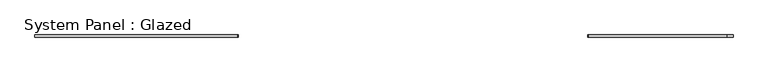
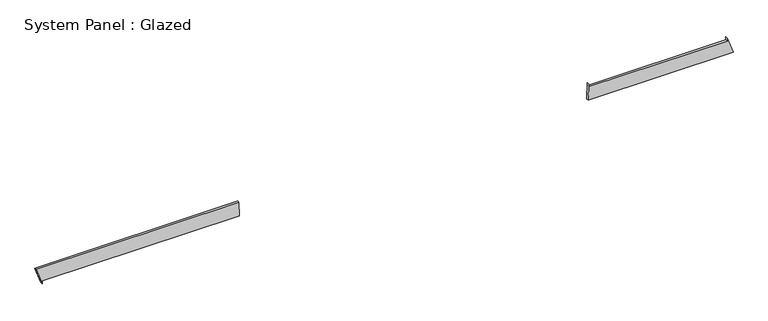
"""IFC4 building model written with IfcOpenShell, lengths in millimetres: plate geometry, System Panel : Glazed."""

import ifcopenshell
import ifcopenshell.guid

model = None  # the IFC model being written
_history = None  # IfcOwnerHistory: only IFC2X3 demands one
_inside = {}  # id of a spatial element -> (the spatial element, [elements in it])
_under = {}  # id of a project, library or spatial element -> (it, [spatial elements below it])
_declared = {}  # id of a project -> (the project, [libraries it declares])
_typed = {}  # id of a type object -> (the type object, [elements of that type])
_made_of = {}  # id of a material, layer set ... -> (it, [elements and type objects made of it])


def new_model(schema):
    """Start an empty IFC model of exactly this schema.

    Asked for "IFC4X3", IfcOpenShell would pick the latest addendum, in which some entities
    have other attributes; the version numbers below select the first issue.
    IFC2X3 requires an IfcOwnerHistory on every rooted entity: one is made here for all.
    """
    global model, _history
    if schema == "IFC4X3":
        model = ifcopenshell.file(schema_version=(4, 3, 0, 0))
    else:
        model = ifcopenshell.file(schema=schema)
    _inside.clear()
    _under.clear()
    _declared.clear()
    _typed.clear()
    _made_of.clear()
    _history = None
    if model.schema == "IFC2X3":
        org = make("IfcOrganization", Name="unknown")
        user = make(
            "IfcPersonAndOrganization",
            ThePerson=make("IfcPerson", FamilyName="unknown"),
            TheOrganization=org,
        )
        app = make(
            "IfcApplication",
            ApplicationDeveloper=org,
            Version="unknown",
            ApplicationFullName="unknown",
            ApplicationIdentifier="unknown",
        )
        _history = make(
            "IfcOwnerHistory",
            OwningUser=user,
            OwningApplication=app,
            ChangeAction="ADDED",
            CreationDate=0,
        )
    return model


def make(cls, **values):
    """One entity of the class cls with the attributes given. An attribute that is None is left unset."""
    return model.create_entity(
        cls, **{name: value for name, value in values.items() if value is not None}
    )


def rooted(cls, **values):
    """An entity with a GlobalId (a new one), such as an element, a storey or a relation."""
    return make(cls, GlobalId=ifcopenshell.guid.new(), OwnerHistory=_history, **values)


def si_unit(unit_type, name, prefix=None):
    """IfcSIUnit, for example si_unit("LENGTHUNIT", "METRE", prefix="MILLI")."""
    return make("IfcSIUnit", UnitType=unit_type, Prefix=prefix, Name=name)


def assignment(units):
    """IfcUnitAssignment: the units of a project."""
    return None if units is None else make("IfcUnitAssignment", Units=units)


def point(xyz):
    """IfcCartesianPoint."""
    return None if xyz is None else make("IfcCartesianPoint", Coordinates=xyz)


def direction(xyz):
    """IfcDirection."""
    return None if xyz is None else make("IfcDirection", DirectionRatios=xyz)


def frame(location, z_axis=None, x_axis=None):
    """IfcAxis2Placement3D, a coordinate frame: its origin and axes. An axis left out is left unset."""
    return make(
        "IfcAxis2Placement3D",
        Location=point(location),
        Axis=direction(z_axis),
        RefDirection=direction(x_axis),
    )


def origin():
    """The frame at (0, 0, 0) with its axes left unset."""
    return frame((0.0, 0.0, 0.0))


def place(relative_to, where):
    """IfcLocalPlacement: puts the frame where relative to a parent placement (None: the world)."""
    return make(
        "IfcLocalPlacement", PlacementRelTo=relative_to, RelativePlacement=where
    )


def context(
    kind, dimensions, precision=None, world=None, true_north=None, identifier=None
):
    """IfcGeometricRepresentationContext, for example the 3D "Model" context."""
    return make(
        "IfcGeometricRepresentationContext",
        ContextIdentifier=identifier,
        ContextType=kind,
        CoordinateSpaceDimension=dimensions,
        Precision=precision,
        WorldCoordinateSystem=world,
        TrueNorth=true_north,
    )


def project(units=None, contexts=None):
    """IfcProject with its units and contexts."""
    return rooted(
        "IfcProject",
        Name="project",
        RepresentationContexts=contexts,
        UnitsInContext=assignment(units),
    )


def spatial(cls, under=None, at=None, **own):
    """A site, building, storey or space (cls), placed at a placement, below another one or the project."""
    s = rooted(cls, ObjectPlacement=at, **own)
    if under is not None:
        _under.setdefault(under.id(), (under, []))[1].append(s)
    return s


def polyline(points):
    """IfcPolyline through the points."""
    return make("IfcPolyline", Points=[point(p) for p in points])


def outline(outer, holes=None, kind="AREA"):
    """IfcArbitraryClosedProfileDef: a profile drawn as a closed curve; with holes, ...WithVoids."""
    if holes is None:
        return make("IfcArbitraryClosedProfileDef", ProfileType=kind, OuterCurve=outer)
    return make(
        "IfcArbitraryProfileDefWithVoids",
        ProfileType=kind,
        OuterCurve=outer,
        InnerCurves=holes,
    )


def extrude(swept, where, along, depth):
    """IfcExtrudedAreaSolid: the profile swept, set in the frame where, extruded along a direction by depth."""
    return make(
        "IfcExtrudedAreaSolid",
        SweptArea=swept,
        Position=where,
        ExtrudedDirection=direction(along),
        Depth=depth,
    )


def shape(context_of_items, identifier, shape_type, items):
    """IfcShapeRepresentation: the items that make up one representation, for example the "Body"."""
    return make(
        "IfcShapeRepresentation",
        ContextOfItems=context_of_items,
        RepresentationIdentifier=identifier,
        RepresentationType=shape_type,
        Items=items,
    )


def source(mapping_origin, context_of_items, identifier, shape_type, items):
    """IfcRepresentationMap: a shape defined once, which mapped items show again and again."""
    return make(
        "IfcRepresentationMap",
        MappingOrigin=mapping_origin,
        MappedRepresentation=shape(context_of_items, identifier, shape_type, items),
    )


def transform(
    local_origin,
    x_axis=None,
    y_axis=None,
    z_axis=None,
    scale=None,
    scale2=None,
    scale3=None,
    uniform=True,
):
    """IfcCartesianTransformationOperator3D, or its non-uniform kind. x_axis, y_axis, z_axis: its Axis1, 2, 3."""
    if uniform:
        return make(
            "IfcCartesianTransformationOperator3D",
            Axis1=direction(x_axis),
            Axis2=direction(y_axis),
            LocalOrigin=point(local_origin),
            Scale=scale,
            Axis3=direction(z_axis),
        )
    return make(
        "IfcCartesianTransformationOperator3DnonUniform",
        Axis1=direction(x_axis),
        Axis2=direction(y_axis),
        LocalOrigin=point(local_origin),
        Scale=scale,
        Axis3=direction(z_axis),
        Scale2=scale2,
        Scale3=scale3,
    )


def mapped(mapping_source, mapping_target):
    """IfcMappedItem: shows the shape of a source again, moved by a transform."""
    return make(
        "IfcMappedItem", MappingSource=mapping_source, MappingTarget=mapping_target
    )


def made_of(thing, what):
    """Note that an element or type object is made of a material, layer set ...; save() writes the relation."""
    if what is not None:
        _made_of.setdefault(what.id(), (what, []))[1].append(thing)
    return thing


def element(
    cls,
    number,
    at=None,
    inside=None,
    cuts=None,
    type_object=None,
    material=None,
    context=None,
    identifier="Body",
    shape_type=None,
    held_by="IfcProductDefinitionShape",
    body=None,
    shapes=None,
    **own,
):
    """One element of the class cls, such as IfcWall. Its Tag is "e" and its number.

    at: its placement. inside: the storey or other place that contains it. cuts: it is an
    opening in that element (IfcRelVoidsElement). A single representation is given by context,
    identifier, shape_type and body (its items); several are given by shapes. held_by: the class
    of the entity that holds the representations. save() writes the other relations.
    """
    e = rooted(cls, Tag="e%d" % number, ObjectPlacement=at, **own)
    if body is not None:
        shapes = [shape(context, identifier, shape_type, body)]
    if shapes is not None:
        e.Representation = make(held_by, Representations=shapes)
    if inside is not None:
        _inside.setdefault(inside.id(), (inside, []))[1].append(e)
    if cuts is not None:
        rooted(
            "IfcRelVoidsElement", RelatingBuildingElement=cuts, RelatedOpeningElement=e
        )
    if type_object is not None:
        _typed.setdefault(type_object.id(), (type_object, []))[1].append(e)
    return made_of(e, material)


def aggregate(whole, parts):
    """IfcRelAggregates: a whole, such as a stair, and the parts it consists of."""
    return rooted("IfcRelAggregates", RelatingObject=whole, RelatedObjects=parts)


def save(model, path):
    """Write the relations noted so far, then the file.

    IfcRelAggregates (storeys below a building ...), IfcRelContainedInSpatialStructure (elements
    in a storey), IfcRelDefinesByType, IfcRelAssociatesMaterial and IfcRelDeclares: one each for
    every whole, place, type object, material and project.
    """
    for whole, parts in _under.values():
        aggregate(whole, parts)
    for where, things in _inside.values():
        rooted(
            "IfcRelContainedInSpatialStructure",
            RelatedElements=things,
            RelatingStructure=where,
        )
    for kind, things in _typed.values():
        rooted("IfcRelDefinesByType", RelatedObjects=things, RelatingType=kind)
    for what, things in _made_of.values():
        rooted("IfcRelAssociatesMaterial", RelatedObjects=things, RelatingMaterial=what)
    for by, libraries in _declared.values():
        rooted("IfcRelDeclares", RelatingContext=by, RelatedDefinitions=libraries)
    model.write(path)


def system_panel_glazed_8560ee69(model_context):
    return source(origin(), model_context, "Body", "SweptSolid", [
        extrude(outline(polyline([(0.0, -3957.3100251), (35.3553391, -3957.3100251), (35.3553391, -1681.6472536), (199.0311077, -1684.9000765), (198.9981604, -4026.9402223), (0.0, -3957.3100251)])), frame((0.0, -49.5, 0.0), z_axis=(0.0, 1.0, 0.0), x_axis=(0.0, 0.0, 1.0)), (0.0, 0.0, 1.0), 25.0),
        extrude(outline(polyline([(35.3553391, 2351.2150268), (35.3553391, 4026.9402223), (234.465824, 3957.5777852), (199.110485, 3957.5782826), (199.0879655, 2356.7975845), (234.4433046, 2356.7970871), (35.3553391, 2351.2150268)])), frame((0.0, -49.5, 0.0), z_axis=(0.0, 1.0, 0.0), x_axis=(0.0, 0.0, 1.0)), (0.0, 0.0, 1.0), 25.0),
    ])


if __name__ == "__main__":
    model = new_model("IFC4")
    model_context = context("Model", 3, world=origin())
    ifc_project = project(units=[si_unit("LENGTHUNIT", "METRE", prefix="MILLI")], contexts=[model_context])
    site = spatial("IfcSite", under=ifc_project)
    building = spatial("IfcBuilding", under=site)
    placement = place(None, origin())
    system_panel_glazed_shape = system_panel_glazed_8560ee69(model_context)
    element("IfcPlate", 1, ObjectType="System Panel : Glazed", at=placement, inside=building, context=model_context, shape_type="MappedRepresentation", body=[
        mapped(system_panel_glazed_shape, transform((0.0, 0.0, 0.0), x_axis=(1.0, 0.0, 0.0), y_axis=(0.0, 1.0, 0.0), z_axis=(0.0, 0.0, 1.0))),
    ])
    save(model, "model.ifc")

# Revit data of these elements
# Element 1 (IfcPlate, "System Panel : Glazed")
#   Materials on its faces: "Glass"
# Materials
#   "Glass": class "Glass", colour RGB 218 227 224, transparency 0.85, Description = "Soda Lime Glass", Cost = 0
